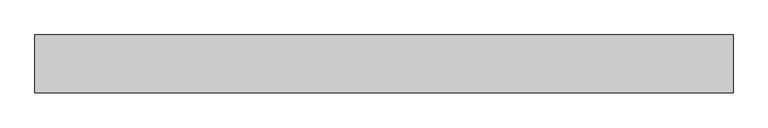
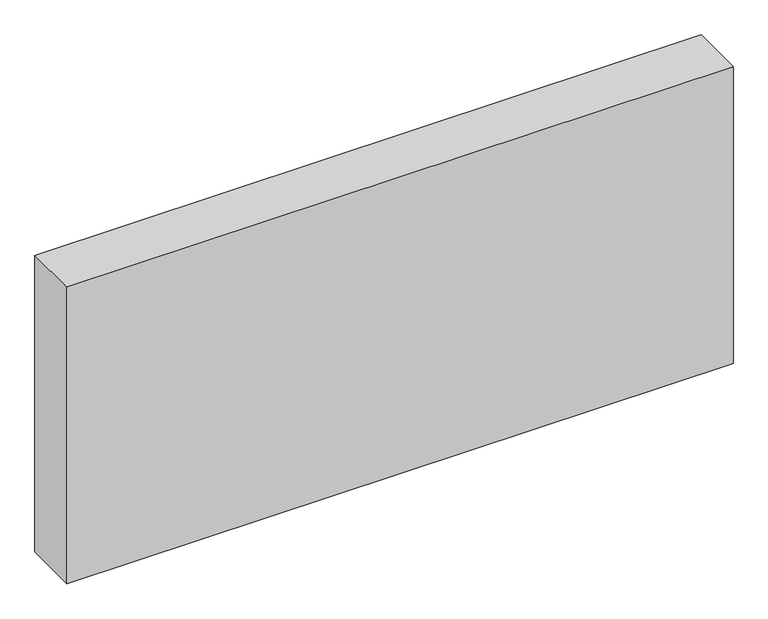
"""IFC4 building model written with IfcOpenShell, lengths in millimetres: proxy geometry, Generic Models 7:Generic Models 1:5:Generic Models 1:5 : Generic Models 7:Generic Models 1:337419:13 : Generic Models 7:Generic Models 1:5:Generic Models 1:5 : Generic Models 7:Generic Models 1:337419:311462."""

from ifc_helpers import new_model, si_unit, frame, origin, place, context, project, spatial, polyline, outline, extrude, source, transform, mapped, element, save


def generic_models_fdadf2c7(model_context):
    return source(origin(), model_context, "Body", "SweptSolid", [
        extrude(outline(polyline([(572897.3867239, -578799.0788841), (572897.3867239, -578999.1038841), (570490.7367239, -578999.1038841), (570490.7367239, -578799.0788841), (572897.3867239, -578799.0788841)])), frame((0.0, 0.0, 1311.0765625), z_axis=(0.0, 0.0, 1.0), x_axis=(1.0, 0.0, 0.0)), (0.0, 0.0, 1.0), 1133.871875),
    ])


if __name__ == "__main__":
    model = new_model("IFC4")
    model_context = context("Model", 3, world=origin())
    ifc_project = project(units=[si_unit("LENGTHUNIT", "METRE", prefix="MILLI")], contexts=[model_context])
    site = spatial("IfcSite", under=ifc_project)
    building = spatial("IfcBuilding", under=site)
    placement = place(None, origin())
    generic_models_shape = generic_models_fdadf2c7(model_context)
    element("IfcBuildingElementProxy", 1, Name="Generic Models 7:Generic Models 1:5:Generic Models 1:5 : Generic Models 7:Generic Models 1:337419:13 : Generic Models 7:Generic Models 1:5:Generic Models 1:5 : Generic Models 7:Generic Models 1:337419:311462", ObjectType="Generic Models 7:Generic Models 1:5:Generic Models 1:5 : Generic Models 7:Generic Models 1:337419:13 : Generic Models 7:Generic Models 1:5:Generic Models 1:5 : Generic Models 7:Generic Models 1:337419:311462", at=placement, inside=building, context=model_context, shape_type="MappedRepresentation", body=[
        mapped(generic_models_shape, transform((0.0, 0.0, 0.0), x_axis=(1.0, 0.0, 0.0), y_axis=(0.0, 1.0, 0.0), z_axis=(0.0, 0.0, 1.0))),
    ])
    save(model, "model.ifc")

# Revit data of these elements
# Type "Generic Models 7:Generic Models 1:5:Generic Models 1:5 : Generic Models 7:Generic Models 1:337419:13 : Generic Models 7:Generic Models 1:5:Generic Models 1:5 : Generic Models 7:Generic Models 1:337419:311462"
#   NameOverride = "Generic Models 7:Generic Models 1:5:Generic Models 1:5 : Generic Models 7:Generic Models 1:337419:311462"
#   ObjectTypeOverride = "Generic Models 1:5 : Generic Models 7:Generic Models 1:337419"
#   Reference = "Generic Models 1"
#   Tag = "311462"
# Element 1 (IfcBuildingElementProxy, "Generic Models 7:Generic Models 1:5:Generic Models 1:5 : Generic Models 7:Generic Models 1:337419:13 : Generic Models 7:Generic Models 1:5:Generic Models 1:5 : Generic Models 7:Generic Models 1:337419:311462")
#   Materials on its faces: "Foiled faced Batt Insulation"
# Materials
#   "Foiled faced Batt Insulation": class "Unassigned", colour RGB 225 232 183, transparency 0, Cost = 0
